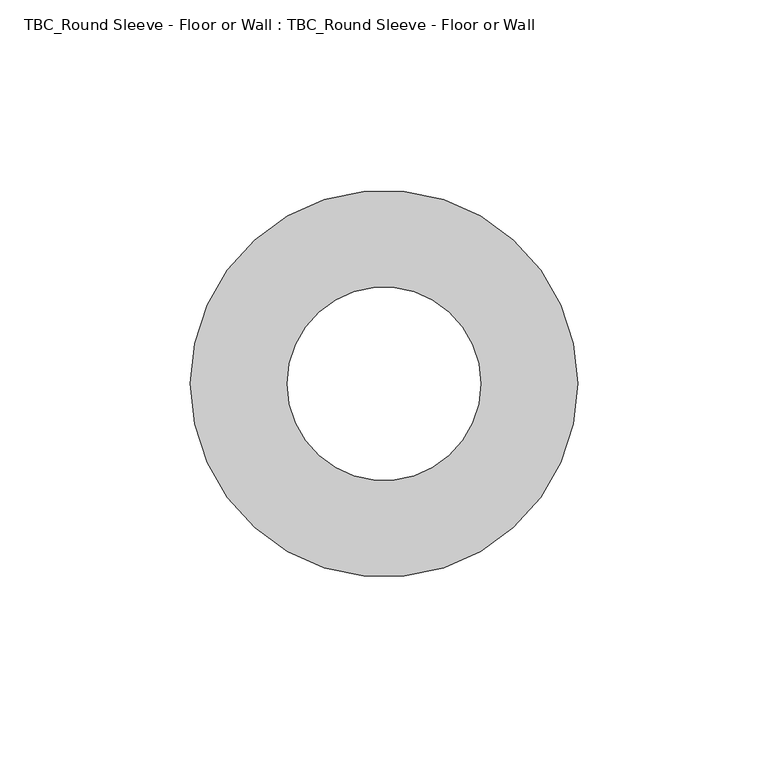
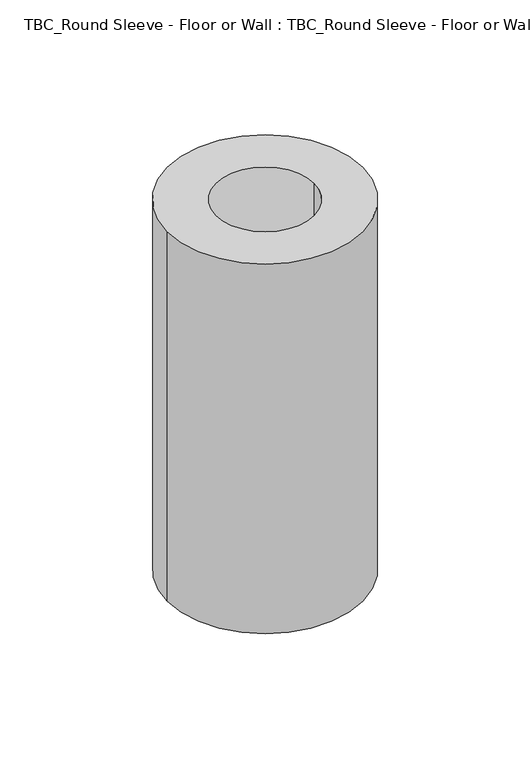
"""IFC4 building model written with IfcOpenShell, lengths in millimetres: proxy geometry, TBC_Round Sleeve - Floor or Wall : TBC_Round Sleeve - Floor or Wall."""

from ifc_helpers import new_model, si_unit, point, frame, origin, origin_2d, place, context, project, spatial, circle_curve, trimmed, segment, composite_curve, outline, extrude, source, transform, mapped, element, save


def tbc_round_sleeve_floor_or_wall_tbc_round_sleeve_floor_or_a2b5493d(model_context):
    return source(origin(), model_context, "Body", "SweptSolid", [
        extrude(outline(composite_curve([segment(trimmed(circle_curve(origin_2d(), 50.8), [point((-50.8, 0.0))], [point((50.8, 0.0))], False, "CARTESIAN"), True, "CONTINUOUS"), segment(trimmed(circle_curve(origin_2d(), 50.8), [point((50.8, 0.0))], [point((-50.8, 0.0))], False, "CARTESIAN"), True, "CONTINUOUS")], self_intersect=False), holes=[composite_curve([segment(trimmed(circle_curve(origin_2d(), 25.4), [point((-25.4, 0.0))], [point((25.4, 0.0))], True, "CARTESIAN"), True, "CONTINUOUS"), segment(trimmed(circle_curve(origin_2d(), 25.4), [point((25.4, 0.0))], [point((-25.4, 0.0))], True, "CARTESIAN"), True, "CONTINUOUS")], self_intersect=False)]), frame((0.0, 0.0, -203.2), z_axis=(0.0, 0.0, 1.0), x_axis=(1.0, 0.0, 0.0)), (0.0, 0.0, 1.0), 203.2),
    ])


if __name__ == "__main__":
    model = new_model("IFC4")
    model_context = context("Model", 3, world=origin())
    ifc_project = project(units=[si_unit("LENGTHUNIT", "METRE", prefix="MILLI")], contexts=[model_context])
    site = spatial("IfcSite", under=ifc_project)
    building = spatial("IfcBuilding", under=site)
    placement = place(None, origin())
    tbc_round_sleeve_floor_or_wall_tbc_round_sleeve_floor_or_shape = tbc_round_sleeve_floor_or_wall_tbc_round_sleeve_floor_or_a2b5493d(model_context)
    element("IfcBuildingElementProxy", 1, Name="TBC_Round Sleeve - Floor or Wall : TBC_Round Sleeve - Floor or Wall", ObjectType="TBC_Round Sleeve - Floor or Wall : TBC_Round Sleeve - Floor or Wall", at=placement, inside=building, context=model_context, shape_type="MappedRepresentation", body=[
        mapped(tbc_round_sleeve_floor_or_wall_tbc_round_sleeve_floor_or_shape, transform((0.0, 0.0, 0.0), x_axis=(1.0, 0.0, 0.0), y_axis=(0.0, 1.0, 0.0), z_axis=(0.0, 0.0, 1.0))),
    ])
    save(model, "model.ifc")

# Revit data of these elements
# Type "TBC_Round Sleeve - Floor or Wall : TBC_Round Sleeve - Floor or Wall"
#   Tag Dimension [instance default] = ""
#   MEP Type [instance default] = ""
#   MEP Element [instance default] = ""
#   MEP Category [instance default] = ""
#   Host Element Type [instance default] = ""
#   Host Element Id [instance default] = ""
#   Host Element Category [instance default] = ""
#   Control Line Y [instance default] = ""
#   Control Line X [instance default] = ""
#   Sleeve Radius [instance default] = 1' - 0"
#   Sleeve Edge [instance default] = 1' - 2"
#   Sleeve Depth [instance default] = 3' - 0"
#   Distance Y [instance default] = 0' - 0"
#   Distance X [instance default] = 0' - 0"
#   Default Elevation = 0
# Element 1 (IfcBuildingElementProxy, "TBC_Round Sleeve - Floor or Wall : TBC_Round Sleeve - Floor or Wall")
#   Tag Dimension = "2\"ø"
#   MEP Type = "Mechanical-CWR"
#   MEP Element = "866065"
#   MEP Category = "Pipe"
#   Host Element Type = "8\" Plank"
#   Host Element Id = "732720"
#   Host Element Category = "Floors"
#   Sleeve Radius = 0' - 2"
#   Sleeve Edge = 0' - 4"
#   Sleeve Depth = 0' - 8"
